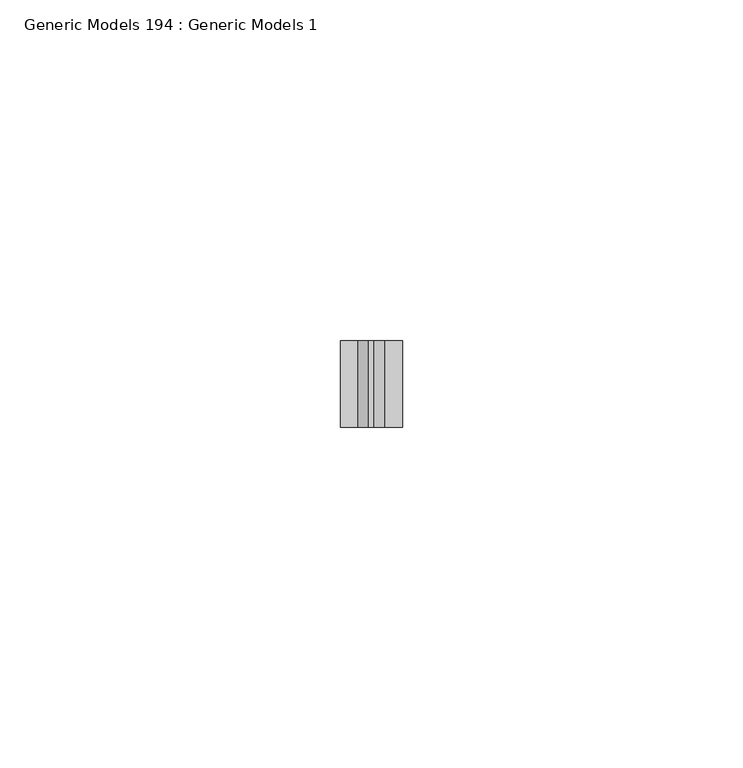
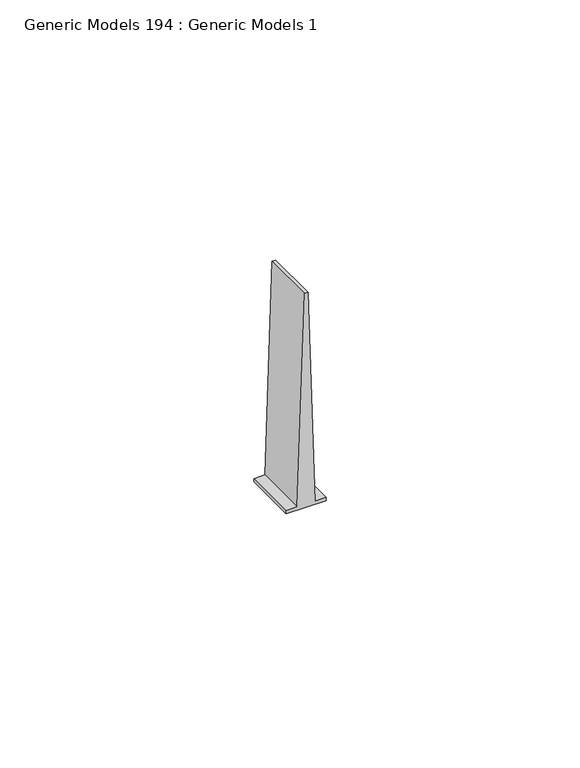
"""IFC4 building model written with IfcOpenShell, lengths in millimetres: proxy geometry, Generic Models 194 : Generic Models 1."""

from ifc_helpers import new_model, si_unit, frame, origin, place, context, project, spatial, polyline, outline, extrude, source, transform, mapped, element, save


def generic_models_194_generic_models_1_34d9de7f(model_context):
    return source(origin(), model_context, "Body", "SweptSolid", [
        extrude(outline(polyline([(2455.06875, 49733.4159), (2455.06875, 49742.5091), (2455.8625, 49742.5091), (2455.8625, 49739.9592364), (2506.6625, 49738.3618473), (2506.6625, 49737.5631527), (2455.8625, 49735.9657636), (2455.8625, 49733.4159), (2455.06875, 49733.4159)])), frame((0.0, 565.15, 0.0), z_axis=(0.0, 1.0, 0.0), x_axis=(0.0, 0.0, 1.0)), (0.0, 0.0, 1.0), 12.7),
    ])


if __name__ == "__main__":
    model = new_model("IFC4")
    model_context = context("Model", 3, world=origin())
    ifc_project = project(units=[si_unit("LENGTHUNIT", "METRE", prefix="MILLI")], contexts=[model_context])
    site = spatial("IfcSite", under=ifc_project)
    building = spatial("IfcBuilding", under=site)
    placement = place(None, origin())
    generic_models_194_generic_models_1_shape = generic_models_194_generic_models_1_34d9de7f(model_context)
    element("IfcBuildingElementProxy", 1, Name="Generic Models 194 : Generic Models 1", ObjectType="Generic Models 194 : Generic Models 1", at=placement, inside=building, context=model_context, shape_type="MappedRepresentation", body=[
        mapped(generic_models_194_generic_models_1_shape, transform((0.0, 0.0, 0.0), x_axis=(1.0, 0.0, 0.0), y_axis=(0.0, 1.0, 0.0), z_axis=(0.0, 0.0, 1.0))),
    ])
    save(model, "model.ifc")

# Revit data of these elements
# Element 1 (IfcBuildingElementProxy, "Generic Models 194 : Generic Models 1")
#   Materials on its faces: "METAL RUNNER CHANNEL; FASTEN @ 24\" O.C."
# Materials
#   "METAL RUNNER CHANNEL; FASTEN @ 24\" O.C.": class "Unassigned", colour RGB 210 209 208, transparency 0, Keynote = "M05121300.02", Cost = 0
